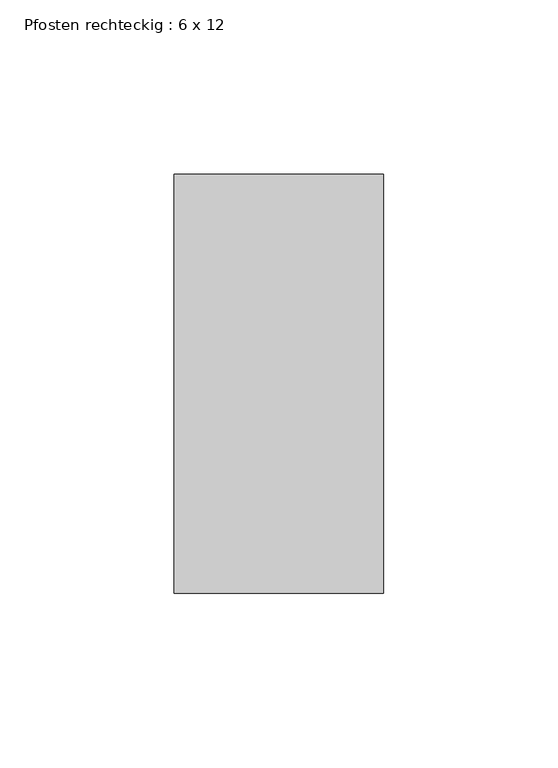
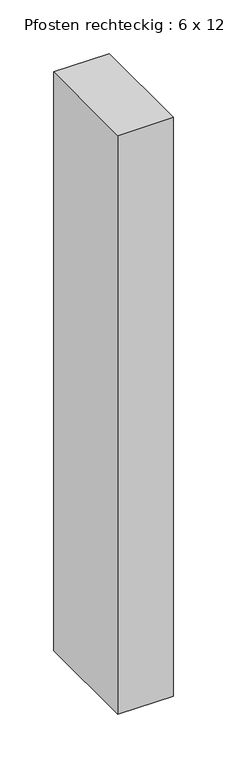
"""IFC4 building model written with IfcOpenShell, lengths in millimetres: member geometry, Pfosten rechteckig : 6 x 12."""

from ifc_helpers import new_model, si_unit, frame, origin, place, context, project, spatial, polyline, outline, extrude, source, transform, mapped, element, save


def pfosten_rechteckig_6_x_12_e841a96c(model_context):
    return source(origin(), model_context, "Body", "SweptSolid", [
        extrude(outline(polyline([(30.0, 60.0), (30.0, -60.0), (-30.0, -60.0), (-30.0, 60.0), (30.0, 60.0)])), frame((0.0, 0.0, -660.287322), z_axis=(0.0, 0.0, 1.0), x_axis=(1.0, 0.0, 0.0)), (0.0, 0.0, 1.0), 660.287322),
    ])


if __name__ == "__main__":
    model = new_model("IFC4")
    model_context = context("Model", 3, world=origin())
    ifc_project = project(units=[si_unit("LENGTHUNIT", "METRE", prefix="MILLI")], contexts=[model_context])
    site = spatial("IfcSite", under=ifc_project)
    building = spatial("IfcBuilding", under=site)
    placement = place(None, origin())
    pfosten_rechteckig_6_x_12_shape = pfosten_rechteckig_6_x_12_e841a96c(model_context)
    element("IfcMember", 1, ObjectType="Pfosten rechteckig : 6 x 12", at=placement, inside=building, context=model_context, shape_type="MappedRepresentation", body=[
        mapped(pfosten_rechteckig_6_x_12_shape, transform((0.0, 0.0, 0.0), x_axis=(1.0, 0.0, 0.0), y_axis=(0.0, 1.0, 0.0), z_axis=(0.0, 0.0, 1.0))),
    ])
    save(model, "model.ifc")

# Revit data of these elements
# Type "Pfosten rechteckig : 6 x 12"
#   built-in parameter 1007304 = 0.393701 (stored number, unit not read)
#   built-in parameter 1007301 = 0.0984252 (stored number, unit not read)
#   built-in parameter 1007300 = 0.0984252 (stored number, unit not read)
# Element 1 (IfcMember, "Pfosten rechteckig : 6 x 12")
#   Materials on its faces: "Metall - verzinkt"
# Materials
#   "Metall - verzinkt": class "Allgemeines", colour RGB 200 200 200, transparency 0, Cost = 0
